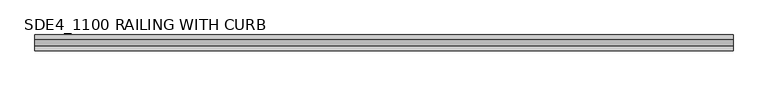
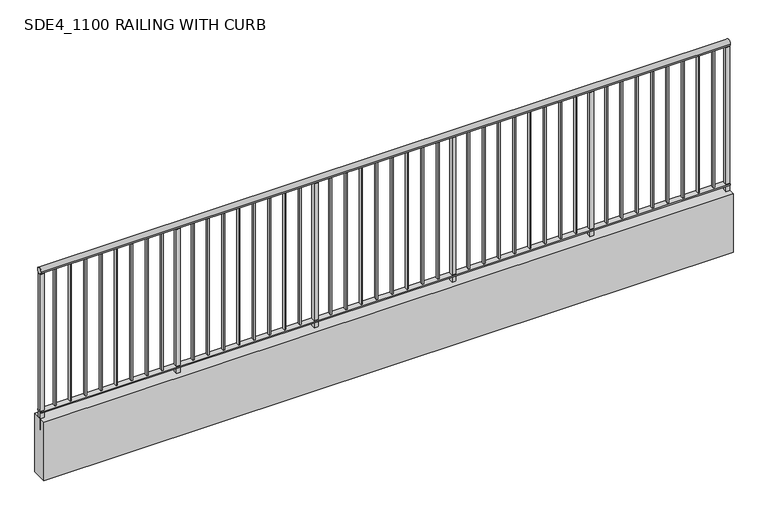
"""IFC4 building model written with IfcOpenShell, lengths in millimetres: railing geometry, SDE4_1100 RAILING WITH CURB."""

from ifc_helpers import new_model, si_unit, point, frame, frame_2d, origin, place, context, project, spatial, polyline, circle_curve, trimmed, segment, composite_curve, outline, extrude, source, transform, mapped, element, save


def sde4_1100_railing_with_curb_a3b336ef(model_context):
    return source(origin(), model_context, "Body", "SweptSolid", [
        extrude(outline(composite_curve([segment(trimmed(circle_curve(frame_2d((27350.4, 131550.0)), 20.0), [point((27370.4, 131550.0))], [point((27330.4, 131550.0))], False, "CARTESIAN"), True, "CONTINUOUS"), segment(trimmed(circle_curve(frame_2d((27350.4, 131550.0)), 20.0), [point((27330.4, 131550.0))], [point((27370.4, 131550.0))], False, "CARTESIAN"), True, "CONTINUOUS")], self_intersect=False)), frame((71847.6057616, 0.0, 0.0), z_axis=(1.0, 0.0, 0.0), x_axis=(0.0, 1.0, 0.0)), (0.0, 0.0, 1.0), 4452.3942384),
        extrude(outline(polyline([(71847.6057616, 27331.4), (71847.6057616, 27369.4), (76300.0, 27369.4), (76300.0, 27331.4), (71847.6057616, 27331.4)])), frame((0.0, 0.0, 130586.0), z_axis=(0.0, 0.0, 1.0), x_axis=(1.0, 0.0, 0.0)), (0.0, 0.0, 1.0), 9.0),
        extrude(outline(polyline([(71847.6057616, 27300.0), (71847.6057616, 27400.0), (76300.0, 27400.0), (76300.0, 27300.0), (71847.6057616, 27300.0)])), frame((0.0, 0.0, 130145.0), z_axis=(0.0, 0.0, 1.0), x_axis=(1.0, 0.0, 0.0)), (0.0, 0.0, 1.0), 400.0),
        extrude(outline(polyline([(76196.5579058, 27341.4), (76196.5579058, 27359.4), (76205.5579058, 27359.4), (76205.5579058, 27341.4), (76196.5579058, 27341.4)])), frame((0.0, 0.0, 130595.0), z_axis=(0.0, 0.0, 1.0), x_axis=(1.0, 0.0, 0.0)), (0.0, 0.0, 1.0), 935.0),
        extrude(outline(polyline([(76097.6158116, 27341.4), (76097.6158116, 27359.4), (76106.6158116, 27359.4), (76106.6158116, 27341.4), (76097.6158116, 27341.4)])), frame((0.0, 0.0, 130595.0), z_axis=(0.0, 0.0, 1.0), x_axis=(1.0, 0.0, 0.0)), (0.0, 0.0, 1.0), 935.0),
        extrude(outline(polyline([(75998.6737174, 27341.4), (75998.6737174, 27359.4), (76007.6737174, 27359.4), (76007.6737174, 27341.4), (75998.6737174, 27341.4)])), frame((0.0, 0.0, 130595.0), z_axis=(0.0, 0.0, 1.0), x_axis=(1.0, 0.0, 0.0)), (0.0, 0.0, 1.0), 935.0),
        extrude(outline(polyline([(75899.7316233, 27341.4), (75899.7316233, 27359.4), (75908.7316233, 27359.4), (75908.7316233, 27341.4), (75899.7316233, 27341.4)])), frame((0.0, 0.0, 130595.0), z_axis=(0.0, 0.0, 1.0), x_axis=(1.0, 0.0, 0.0)), (0.0, 0.0, 1.0), 935.0),
        extrude(outline(polyline([(75800.7895291, 27341.4), (75800.7895291, 27359.4), (75809.7895291, 27359.4), (75809.7895291, 27341.4), (75800.7895291, 27341.4)])), frame((0.0, 0.0, 130595.0), z_axis=(0.0, 0.0, 1.0), x_axis=(1.0, 0.0, 0.0)), (0.0, 0.0, 1.0), 935.0),
        extrude(outline(polyline([(75701.8474349, 27341.4), (75701.8474349, 27359.4), (75710.8474349, 27359.4), (75710.8474349, 27341.4), (75701.8474349, 27341.4)])), frame((0.0, 0.0, 130595.0), z_axis=(0.0, 0.0, 1.0), x_axis=(1.0, 0.0, 0.0)), (0.0, 0.0, 1.0), 935.0),
        extrude(outline(polyline([(75602.9053407, 27341.4), (75602.9053407, 27359.4), (75611.9053407, 27359.4), (75611.9053407, 27341.4), (75602.9053407, 27341.4)])), frame((0.0, 0.0, 130595.0), z_axis=(0.0, 0.0, 1.0), x_axis=(1.0, 0.0, 0.0)), (0.0, 0.0, 1.0), 935.0),
        extrude(outline(polyline([(75503.9632465, 27341.4), (75503.9632465, 27359.4), (75512.9632465, 27359.4), (75512.9632465, 27341.4), (75503.9632465, 27341.4)])), frame((0.0, 0.0, 130595.0), z_axis=(0.0, 0.0, 1.0), x_axis=(1.0, 0.0, 0.0)), (0.0, 0.0, 1.0), 935.0),
        extrude(outline(polyline([(75397.0211523, 27337.9), (75397.0211523, 27362.9), (75422.0211523, 27362.9), (75422.0211523, 27337.9), (75397.0211523, 27337.9)])), frame((0.0, 0.0, 130545.0), z_axis=(0.0, 0.0, 1.0), x_axis=(1.0, 0.0, 0.0)), (0.0, 0.0, 1.0), 985.0),
        extrude(outline(polyline([(75306.0790581, 27341.4), (75306.0790581, 27359.4), (75315.0790581, 27359.4), (75315.0790581, 27341.4), (75306.0790581, 27341.4)])), frame((0.0, 0.0, 130595.0), z_axis=(0.0, 0.0, 1.0), x_axis=(1.0, 0.0, 0.0)), (0.0, 0.0, 1.0), 935.0),
        extrude(outline(polyline([(75207.136964, 27341.4), (75207.136964, 27359.4), (75216.136964, 27359.4), (75216.136964, 27341.4), (75207.136964, 27341.4)])), frame((0.0, 0.0, 130595.0), z_axis=(0.0, 0.0, 1.0), x_axis=(1.0, 0.0, 0.0)), (0.0, 0.0, 1.0), 935.0),
        extrude(outline(polyline([(75108.1948698, 27341.4), (75108.1948698, 27359.4), (75117.1948698, 27359.4), (75117.1948698, 27341.4), (75108.1948698, 27341.4)])), frame((0.0, 0.0, 130595.0), z_axis=(0.0, 0.0, 1.0), x_axis=(1.0, 0.0, 0.0)), (0.0, 0.0, 1.0), 935.0),
        extrude(outline(polyline([(75009.2527756, 27341.4), (75009.2527756, 27359.4), (75018.2527756, 27359.4), (75018.2527756, 27341.4), (75009.2527756, 27341.4)])), frame((0.0, 0.0, 130595.0), z_axis=(0.0, 0.0, 1.0), x_axis=(1.0, 0.0, 0.0)), (0.0, 0.0, 1.0), 935.0),
        extrude(outline(polyline([(74910.3106814, 27341.4), (74910.3106814, 27359.4), (74919.3106814, 27359.4), (74919.3106814, 27341.4), (74910.3106814, 27341.4)])), frame((0.0, 0.0, 130595.0), z_axis=(0.0, 0.0, 1.0), x_axis=(1.0, 0.0, 0.0)), (0.0, 0.0, 1.0), 935.0),
        extrude(outline(polyline([(74811.3685872, 27341.4), (74811.3685872, 27359.4), (74820.3685872, 27359.4), (74820.3685872, 27341.4), (74811.3685872, 27341.4)])), frame((0.0, 0.0, 130595.0), z_axis=(0.0, 0.0, 1.0), x_axis=(1.0, 0.0, 0.0)), (0.0, 0.0, 1.0), 935.0),
        extrude(outline(polyline([(74712.426493, 27341.4), (74712.426493, 27359.4), (74721.426493, 27359.4), (74721.426493, 27341.4), (74712.426493, 27341.4)])), frame((0.0, 0.0, 130595.0), z_axis=(0.0, 0.0, 1.0), x_axis=(1.0, 0.0, 0.0)), (0.0, 0.0, 1.0), 935.0),
        extrude(outline(polyline([(74613.4843988, 27341.4), (74613.4843988, 27359.4), (74622.4843988, 27359.4), (74622.4843988, 27341.4), (74613.4843988, 27341.4)])), frame((0.0, 0.0, 130595.0), z_axis=(0.0, 0.0, 1.0), x_axis=(1.0, 0.0, 0.0)), (0.0, 0.0, 1.0), 935.0),
        extrude(outline(polyline([(74506.5423047, 27337.9), (74506.5423047, 27362.9), (74531.5423047, 27362.9), (74531.5423047, 27337.9), (74506.5423047, 27337.9)])), frame((0.0, 0.0, 130545.0), z_axis=(0.0, 0.0, 1.0), x_axis=(1.0, 0.0, 0.0)), (0.0, 0.0, 1.0), 985.0),
        extrude(outline(polyline([(74415.6002105, 27341.4), (74415.6002105, 27359.4), (74424.6002105, 27359.4), (74424.6002105, 27341.4), (74415.6002105, 27341.4)])), frame((0.0, 0.0, 130595.0), z_axis=(0.0, 0.0, 1.0), x_axis=(1.0, 0.0, 0.0)), (0.0, 0.0, 1.0), 935.0),
        extrude(outline(polyline([(74316.6581163, 27341.4), (74316.6581163, 27359.4), (74325.6581163, 27359.4), (74325.6581163, 27341.4), (74316.6581163, 27341.4)])), frame((0.0, 0.0, 130595.0), z_axis=(0.0, 0.0, 1.0), x_axis=(1.0, 0.0, 0.0)), (0.0, 0.0, 1.0), 935.0),
        extrude(outline(polyline([(74217.7160221, 27341.4), (74217.7160221, 27359.4), (74226.7160221, 27359.4), (74226.7160221, 27341.4), (74217.7160221, 27341.4)])), frame((0.0, 0.0, 130595.0), z_axis=(0.0, 0.0, 1.0), x_axis=(1.0, 0.0, 0.0)), (0.0, 0.0, 1.0), 935.0),
        extrude(outline(polyline([(74118.7739279, 27341.4), (74118.7739279, 27359.4), (74127.7739279, 27359.4), (74127.7739279, 27341.4), (74118.7739279, 27341.4)])), frame((0.0, 0.0, 130595.0), z_axis=(0.0, 0.0, 1.0), x_axis=(1.0, 0.0, 0.0)), (0.0, 0.0, 1.0), 935.0),
        extrude(outline(polyline([(74019.8318337, 27341.4), (74019.8318337, 27359.4), (74028.8318337, 27359.4), (74028.8318337, 27341.4), (74019.8318337, 27341.4)])), frame((0.0, 0.0, 130595.0), z_axis=(0.0, 0.0, 1.0), x_axis=(1.0, 0.0, 0.0)), (0.0, 0.0, 1.0), 935.0),
        extrude(outline(polyline([(73920.8897395, 27341.4), (73920.8897395, 27359.4), (73929.8897395, 27359.4), (73929.8897395, 27341.4), (73920.8897395, 27341.4)])), frame((0.0, 0.0, 130595.0), z_axis=(0.0, 0.0, 1.0), x_axis=(1.0, 0.0, 0.0)), (0.0, 0.0, 1.0), 935.0),
        extrude(outline(polyline([(73821.9476454, 27341.4), (73821.9476454, 27359.4), (73830.9476454, 27359.4), (73830.9476454, 27341.4), (73821.9476454, 27341.4)])), frame((0.0, 0.0, 130595.0), z_axis=(0.0, 0.0, 1.0), x_axis=(1.0, 0.0, 0.0)), (0.0, 0.0, 1.0), 935.0),
        extrude(outline(polyline([(73723.0055512, 27341.4), (73723.0055512, 27359.4), (73732.0055512, 27359.4), (73732.0055512, 27341.4), (73723.0055512, 27341.4)])), frame((0.0, 0.0, 130595.0), z_axis=(0.0, 0.0, 1.0), x_axis=(1.0, 0.0, 0.0)), (0.0, 0.0, 1.0), 935.0),
        extrude(outline(polyline([(73616.063457, 27337.9), (73616.063457, 27362.9), (73641.063457, 27362.9), (73641.063457, 27337.9), (73616.063457, 27337.9)])), frame((0.0, 0.0, 130545.0), z_axis=(0.0, 0.0, 1.0), x_axis=(1.0, 0.0, 0.0)), (0.0, 0.0, 1.0), 985.0),
        extrude(outline(polyline([(73525.1213628, 27341.4), (73525.1213628, 27359.4), (73534.1213628, 27359.4), (73534.1213628, 27341.4), (73525.1213628, 27341.4)])), frame((0.0, 0.0, 130595.0), z_axis=(0.0, 0.0, 1.0), x_axis=(1.0, 0.0, 0.0)), (0.0, 0.0, 1.0), 935.0),
        extrude(outline(polyline([(73426.1792686, 27341.4), (73426.1792686, 27359.4), (73435.1792686, 27359.4), (73435.1792686, 27341.4), (73426.1792686, 27341.4)])), frame((0.0, 0.0, 130595.0), z_axis=(0.0, 0.0, 1.0), x_axis=(1.0, 0.0, 0.0)), (0.0, 0.0, 1.0), 935.0),
        extrude(outline(polyline([(73327.2371744, 27341.4), (73327.2371744, 27359.4), (73336.2371744, 27359.4), (73336.2371744, 27341.4), (73327.2371744, 27341.4)])), frame((0.0, 0.0, 130595.0), z_axis=(0.0, 0.0, 1.0), x_axis=(1.0, 0.0, 0.0)), (0.0, 0.0, 1.0), 935.0),
        extrude(outline(polyline([(73228.2950802, 27341.4), (73228.2950802, 27359.4), (73237.2950802, 27359.4), (73237.2950802, 27341.4), (73228.2950802, 27341.4)])), frame((0.0, 0.0, 130595.0), z_axis=(0.0, 0.0, 1.0), x_axis=(1.0, 0.0, 0.0)), (0.0, 0.0, 1.0), 935.0),
        extrude(outline(polyline([(73129.3529861, 27341.4), (73129.3529861, 27359.4), (73138.3529861, 27359.4), (73138.3529861, 27341.4), (73129.3529861, 27341.4)])), frame((0.0, 0.0, 130595.0), z_axis=(0.0, 0.0, 1.0), x_axis=(1.0, 0.0, 0.0)), (0.0, 0.0, 1.0), 935.0),
        extrude(outline(polyline([(73030.4108919, 27341.4), (73030.4108919, 27359.4), (73039.4108919, 27359.4), (73039.4108919, 27341.4), (73030.4108919, 27341.4)])), frame((0.0, 0.0, 130595.0), z_axis=(0.0, 0.0, 1.0), x_axis=(1.0, 0.0, 0.0)), (0.0, 0.0, 1.0), 935.0),
        extrude(outline(polyline([(72931.4687977, 27341.4), (72931.4687977, 27359.4), (72940.4687977, 27359.4), (72940.4687977, 27341.4), (72931.4687977, 27341.4)])), frame((0.0, 0.0, 130595.0), z_axis=(0.0, 0.0, 1.0), x_axis=(1.0, 0.0, 0.0)), (0.0, 0.0, 1.0), 935.0),
        extrude(outline(polyline([(72832.5267035, 27341.4), (72832.5267035, 27359.4), (72841.5267035, 27359.4), (72841.5267035, 27341.4), (72832.5267035, 27341.4)])), frame((0.0, 0.0, 130595.0), z_axis=(0.0, 0.0, 1.0), x_axis=(1.0, 0.0, 0.0)), (0.0, 0.0, 1.0), 935.0),
        extrude(outline(polyline([(72725.5846093, 27337.9), (72725.5846093, 27362.9), (72750.5846093, 27362.9), (72750.5846093, 27337.9), (72725.5846093, 27337.9)])), frame((0.0, 0.0, 130545.0), z_axis=(0.0, 0.0, 1.0), x_axis=(1.0, 0.0, 0.0)), (0.0, 0.0, 1.0), 985.0),
        extrude(outline(polyline([(72634.6425151, 27341.4), (72634.6425151, 27359.4), (72643.6425151, 27359.4), (72643.6425151, 27341.4), (72634.6425151, 27341.4)])), frame((0.0, 0.0, 130595.0), z_axis=(0.0, 0.0, 1.0), x_axis=(1.0, 0.0, 0.0)), (0.0, 0.0, 1.0), 935.0),
        extrude(outline(polyline([(72535.7004209, 27341.4), (72535.7004209, 27359.4), (72544.7004209, 27359.4), (72544.7004209, 27341.4), (72535.7004209, 27341.4)])), frame((0.0, 0.0, 130595.0), z_axis=(0.0, 0.0, 1.0), x_axis=(1.0, 0.0, 0.0)), (0.0, 0.0, 1.0), 935.0),
        extrude(outline(polyline([(72436.7583268, 27341.4), (72436.7583268, 27359.4), (72445.7583268, 27359.4), (72445.7583268, 27341.4), (72436.7583268, 27341.4)])), frame((0.0, 0.0, 130595.0), z_axis=(0.0, 0.0, 1.0), x_axis=(1.0, 0.0, 0.0)), (0.0, 0.0, 1.0), 935.0),
        extrude(outline(polyline([(72337.8162326, 27341.4), (72337.8162326, 27359.4), (72346.8162326, 27359.4), (72346.8162326, 27341.4), (72337.8162326, 27341.4)])), frame((0.0, 0.0, 130595.0), z_axis=(0.0, 0.0, 1.0), x_axis=(1.0, 0.0, 0.0)), (0.0, 0.0, 1.0), 935.0),
        extrude(outline(polyline([(72238.8741384, 27341.4), (72238.8741384, 27359.4), (72247.8741384, 27359.4), (72247.8741384, 27341.4), (72238.8741384, 27341.4)])), frame((0.0, 0.0, 130595.0), z_axis=(0.0, 0.0, 1.0), x_axis=(1.0, 0.0, 0.0)), (0.0, 0.0, 1.0), 935.0),
        extrude(outline(polyline([(72139.9320442, 27341.4), (72139.9320442, 27359.4), (72148.9320442, 27359.4), (72148.9320442, 27341.4), (72139.9320442, 27341.4)])), frame((0.0, 0.0, 130595.0), z_axis=(0.0, 0.0, 1.0), x_axis=(1.0, 0.0, 0.0)), (0.0, 0.0, 1.0), 935.0),
        extrude(outline(polyline([(72040.98995, 27341.4), (72040.98995, 27359.4), (72049.98995, 27359.4), (72049.98995, 27341.4), (72040.98995, 27341.4)])), frame((0.0, 0.0, 130595.0), z_axis=(0.0, 0.0, 1.0), x_axis=(1.0, 0.0, 0.0)), (0.0, 0.0, 1.0), 935.0),
        extrude(outline(polyline([(71942.0478558, 27341.4), (71942.0478558, 27359.4), (71951.0478558, 27359.4), (71951.0478558, 27341.4), (71942.0478558, 27341.4)])), frame((0.0, 0.0, 130595.0), z_axis=(0.0, 0.0, 1.0), x_axis=(1.0, 0.0, 0.0)), (0.0, 0.0, 1.0), 935.0),
        extrude(outline(polyline([(76275.0, 27362.9), (76300.0, 27362.9), (76300.0, 27337.9), (76275.0, 27337.9), (76275.0, 27362.9)])), frame((0.0, 0.0, 130470.0), z_axis=(0.0, 0.0, 1.0), x_axis=(1.0, 0.0, 0.0)), (0.0, 0.0, 1.0), 1060.0),
        extrude(outline(polyline([(71847.6057616, 27362.9), (71872.6057616, 27362.9), (71872.6057616, 27337.9), (71847.6057616, 27337.9), (71847.6057616, 27362.9)])), frame((0.0, 0.0, 130470.0), z_axis=(0.0, 0.0, 1.0), x_axis=(1.0, 0.0, 0.0)), (0.0, 0.0, 1.0), 1060.0),
    ])


if __name__ == "__main__":
    model = new_model("IFC4")
    model_context = context("Model", 3, world=origin())
    ifc_project = project(units=[si_unit("LENGTHUNIT", "METRE", prefix="MILLI")], contexts=[model_context])
    site = spatial("IfcSite", under=ifc_project)
    building = spatial("IfcBuilding", under=site)
    placement = place(None, origin())
    sde4_1100_railing_with_curb_shape = sde4_1100_railing_with_curb_a3b336ef(model_context)
    element("IfcRailing", 1, ObjectType="SDE4_1100 RAILING WITH CURB", at=placement, inside=building, context=model_context, shape_type="MappedRepresentation", body=[
        mapped(sde4_1100_railing_with_curb_shape, transform((0.0, 0.0, 0.0), x_axis=(1.0, 0.0, 0.0), y_axis=(0.0, 1.0, 0.0), z_axis=(0.0, 0.0, 1.0))),
    ])
    save(model, "model.ifc")

# Revit data of these elements
# Element 1 (IfcRailing, "SDE4_1100 RAILING WITH CURB")
#   Materials on its faces: "Metal - Steel", "Concrete - Cast-in-Place Concrete"
# Materials
#   "Metal - Steel": class "Metal", colour RGB 247 247 247, transparency 0
#   "Concrete - Cast-in-Place Concrete": class "Concrete", colour RGB 191 178 173, transparency 0, Keynote = "E10/132", Cost = 0
